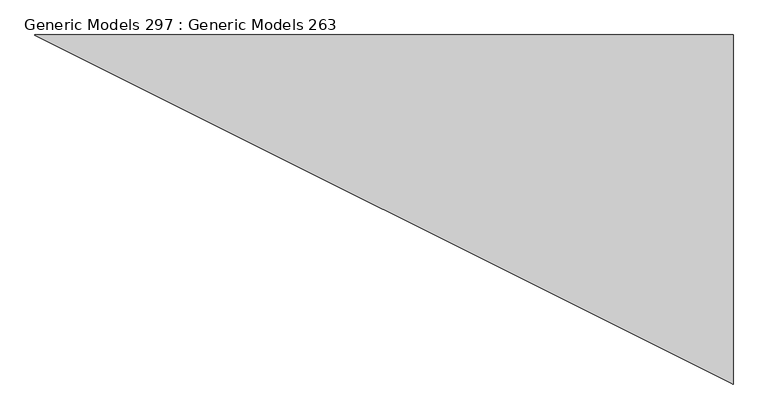
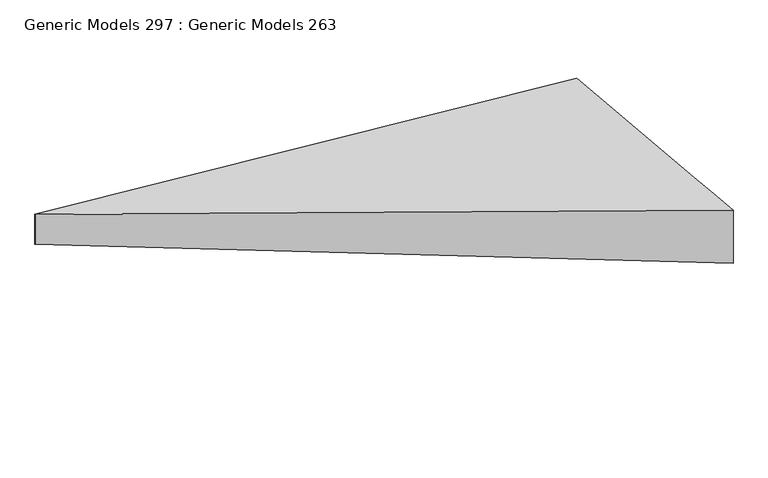
"""IFC4 building model written with IfcOpenShell, lengths in millimetres: proxy geometry, Generic Models 297 : Generic Models 263."""

import ifcopenshell
import ifcopenshell.guid

model = None  # the IFC model being written
_history = None  # IfcOwnerHistory: only IFC2X3 demands one
_inside = {}  # id of a spatial element -> (the spatial element, [elements in it])
_under = {}  # id of a project, library or spatial element -> (it, [spatial elements below it])
_declared = {}  # id of a project -> (the project, [libraries it declares])
_typed = {}  # id of a type object -> (the type object, [elements of that type])
_made_of = {}  # id of a material, layer set ... -> (it, [elements and type objects made of it])


def new_model(schema):
    """Start an empty IFC model of exactly this schema.

    Asked for "IFC4X3", IfcOpenShell would pick the latest addendum, in which some entities
    have other attributes; the version numbers below select the first issue.
    IFC2X3 requires an IfcOwnerHistory on every rooted entity: one is made here for all.
    """
    global model, _history
    if schema == "IFC4X3":
        model = ifcopenshell.file(schema_version=(4, 3, 0, 0))
    else:
        model = ifcopenshell.file(schema=schema)
    _inside.clear()
    _under.clear()
    _declared.clear()
    _typed.clear()
    _made_of.clear()
    _history = None
    if model.schema == "IFC2X3":
        org = make("IfcOrganization", Name="unknown")
        user = make(
            "IfcPersonAndOrganization",
            ThePerson=make("IfcPerson", FamilyName="unknown"),
            TheOrganization=org,
        )
        app = make(
            "IfcApplication",
            ApplicationDeveloper=org,
            Version="unknown",
            ApplicationFullName="unknown",
            ApplicationIdentifier="unknown",
        )
        _history = make(
            "IfcOwnerHistory",
            OwningUser=user,
            OwningApplication=app,
            ChangeAction="ADDED",
            CreationDate=0,
        )
    return model


def make(cls, **values):
    """One entity of the class cls with the attributes given. An attribute that is None is left unset."""
    return model.create_entity(
        cls, **{name: value for name, value in values.items() if value is not None}
    )


def rooted(cls, **values):
    """An entity with a GlobalId (a new one), such as an element, a storey or a relation."""
    return make(cls, GlobalId=ifcopenshell.guid.new(), OwnerHistory=_history, **values)


def si_unit(unit_type, name, prefix=None):
    """IfcSIUnit, for example si_unit("LENGTHUNIT", "METRE", prefix="MILLI")."""
    return make("IfcSIUnit", UnitType=unit_type, Prefix=prefix, Name=name)


def assignment(units):
    """IfcUnitAssignment: the units of a project."""
    return None if units is None else make("IfcUnitAssignment", Units=units)


def point(xyz):
    """IfcCartesianPoint."""
    return None if xyz is None else make("IfcCartesianPoint", Coordinates=xyz)


def direction(xyz):
    """IfcDirection."""
    return None if xyz is None else make("IfcDirection", DirectionRatios=xyz)


def frame(location, z_axis=None, x_axis=None):
    """IfcAxis2Placement3D, a coordinate frame: its origin and axes. An axis left out is left unset."""
    return make(
        "IfcAxis2Placement3D",
        Location=point(location),
        Axis=direction(z_axis),
        RefDirection=direction(x_axis),
    )


def origin():
    """The frame at (0, 0, 0) with its axes left unset."""
    return frame((0.0, 0.0, 0.0))


def place(relative_to, where):
    """IfcLocalPlacement: puts the frame where relative to a parent placement (None: the world)."""
    return make(
        "IfcLocalPlacement", PlacementRelTo=relative_to, RelativePlacement=where
    )


def context(
    kind, dimensions, precision=None, world=None, true_north=None, identifier=None
):
    """IfcGeometricRepresentationContext, for example the 3D "Model" context."""
    return make(
        "IfcGeometricRepresentationContext",
        ContextIdentifier=identifier,
        ContextType=kind,
        CoordinateSpaceDimension=dimensions,
        Precision=precision,
        WorldCoordinateSystem=world,
        TrueNorth=true_north,
    )


def project(units=None, contexts=None):
    """IfcProject with its units and contexts."""
    return rooted(
        "IfcProject",
        Name="project",
        RepresentationContexts=contexts,
        UnitsInContext=assignment(units),
    )


def spatial(cls, under=None, at=None, **own):
    """A site, building, storey or space (cls), placed at a placement, below another one or the project."""
    s = rooted(cls, ObjectPlacement=at, **own)
    if under is not None:
        _under.setdefault(under.id(), (under, []))[1].append(s)
    return s


def shape(context_of_items, identifier, shape_type, items):
    """IfcShapeRepresentation: the items that make up one representation, for example the "Body"."""
    return make(
        "IfcShapeRepresentation",
        ContextOfItems=context_of_items,
        RepresentationIdentifier=identifier,
        RepresentationType=shape_type,
        Items=items,
    )


def source(mapping_origin, context_of_items, identifier, shape_type, items):
    """IfcRepresentationMap: a shape defined once, which mapped items show again and again."""
    return make(
        "IfcRepresentationMap",
        MappingOrigin=mapping_origin,
        MappedRepresentation=shape(context_of_items, identifier, shape_type, items),
    )


def transform(
    local_origin,
    x_axis=None,
    y_axis=None,
    z_axis=None,
    scale=None,
    scale2=None,
    scale3=None,
    uniform=True,
):
    """IfcCartesianTransformationOperator3D, or its non-uniform kind. x_axis, y_axis, z_axis: its Axis1, 2, 3."""
    if uniform:
        return make(
            "IfcCartesianTransformationOperator3D",
            Axis1=direction(x_axis),
            Axis2=direction(y_axis),
            LocalOrigin=point(local_origin),
            Scale=scale,
            Axis3=direction(z_axis),
        )
    return make(
        "IfcCartesianTransformationOperator3DnonUniform",
        Axis1=direction(x_axis),
        Axis2=direction(y_axis),
        LocalOrigin=point(local_origin),
        Scale=scale,
        Axis3=direction(z_axis),
        Scale2=scale2,
        Scale3=scale3,
    )


def mapped(mapping_source, mapping_target):
    """IfcMappedItem: shows the shape of a source again, moved by a transform."""
    return make(
        "IfcMappedItem", MappingSource=mapping_source, MappingTarget=mapping_target
    )


def made_of(thing, what):
    """Note that an element or type object is made of a material, layer set ...; save() writes the relation."""
    if what is not None:
        _made_of.setdefault(what.id(), (what, []))[1].append(thing)
    return thing


def element(
    cls,
    number,
    at=None,
    inside=None,
    cuts=None,
    type_object=None,
    material=None,
    context=None,
    identifier="Body",
    shape_type=None,
    held_by="IfcProductDefinitionShape",
    body=None,
    shapes=None,
    **own,
):
    """One element of the class cls, such as IfcWall. Its Tag is "e" and its number.

    at: its placement. inside: the storey or other place that contains it. cuts: it is an
    opening in that element (IfcRelVoidsElement). A single representation is given by context,
    identifier, shape_type and body (its items); several are given by shapes. held_by: the class
    of the entity that holds the representations. save() writes the other relations.
    """
    e = rooted(cls, Tag="e%d" % number, ObjectPlacement=at, **own)
    if body is not None:
        shapes = [shape(context, identifier, shape_type, body)]
    if shapes is not None:
        e.Representation = make(held_by, Representations=shapes)
    if inside is not None:
        _inside.setdefault(inside.id(), (inside, []))[1].append(e)
    if cuts is not None:
        rooted(
            "IfcRelVoidsElement", RelatingBuildingElement=cuts, RelatedOpeningElement=e
        )
    if type_object is not None:
        _typed.setdefault(type_object.id(), (type_object, []))[1].append(e)
    return made_of(e, material)


def aggregate(whole, parts):
    """IfcRelAggregates: a whole, such as a stair, and the parts it consists of."""
    return rooted("IfcRelAggregates", RelatingObject=whole, RelatedObjects=parts)


def save(model, path):
    """Write the relations noted so far, then the file.

    IfcRelAggregates (storeys below a building ...), IfcRelContainedInSpatialStructure (elements
    in a storey), IfcRelDefinesByType, IfcRelAssociatesMaterial and IfcRelDeclares: one each for
    every whole, place, type object, material and project.
    """
    for whole, parts in _under.values():
        aggregate(whole, parts)
    for where, things in _inside.values():
        rooted(
            "IfcRelContainedInSpatialStructure",
            RelatedElements=things,
            RelatingStructure=where,
        )
    for kind, things in _typed.values():
        rooted("IfcRelDefinesByType", RelatedObjects=things, RelatingType=kind)
    for what, things in _made_of.values():
        rooted("IfcRelAssociatesMaterial", RelatedObjects=things, RelatingMaterial=what)
    for by, libraries in _declared.values():
        rooted("IfcRelDeclares", RelatingContext=by, RelatedDefinitions=libraries)
    model.write(path)


def plane_surface(at):
    """IfcPlane: the flat surface through the origin of the frame at, square to its z axis."""
    return make("IfcPlane", Position=at)


def spline_surface(u_degree, v_degree, points, u_multiplicities, v_multiplicities, u_knots, v_knots, weights=None):
    """IfcBSplineSurfaceWithKnots; with weights, IfcRationalBSplineSurfaceWithKnots. points: one row for each step in u."""
    own = dict(
        UDegree=u_degree,
        VDegree=v_degree,
        ControlPointsList=[[point(p) for p in row] for row in points],
        SurfaceForm="UNSPECIFIED",
        UClosed=False,
        VClosed=False,
        SelfIntersect=False,
        UMultiplicities=u_multiplicities,
        VMultiplicities=v_multiplicities,
        UKnots=u_knots,
        VKnots=v_knots,
        KnotSpec="UNSPECIFIED",
    )
    if weights is None:
        return make("IfcBSplineSurfaceWithKnots", **own)
    return make("IfcRationalBSplineSurfaceWithKnots", WeightsData=weights, **own)


def advanced_brep(points, edges, surfaces, faces):
    """IfcAdvancedBrep: a solid bounded by faces that lie on surfaces and meet in shared edges.

    An edge is (start, end): straight between two places in points (the first is 0);
    or (start, end, curve); or (start, end, curve, False) where it runs against its curve.
    A face is (place in surfaces, loops), or (place, loops, False) where it looks against
    its surface's normal. A loop lists edges by number (the first is 1), with a minus sign
    where the edge is run from its end to its start. The first loop is the outer one.
    """
    corners = [point(p) for p in points]
    vertices = [make("IfcVertexPoint", VertexGeometry=c) for c in corners]
    made = []
    for start, end, *more in edges:
        made.append(
            make(
                "IfcEdgeCurve",
                EdgeStart=vertices[start],
                EdgeEnd=vertices[end],
                EdgeGeometry=more[0] if more else make("IfcPolyline", Points=[corners[start], corners[end]]),
                SameSense=more[1] if len(more) > 1 else True,
            )
        )
    hull = []
    for where, loops, *sense in faces:
        bounds = []
        for j, loop in enumerate(loops):
            ring = [make("IfcOrientedEdge", EdgeElement=made[abs(k) - 1], Orientation=k > 0) for k in loop]
            bounds.append(
                make(
                    "IfcFaceOuterBound" if j == 0 else "IfcFaceBound",
                    Bound=make("IfcEdgeLoop", EdgeList=ring),
                    Orientation=True,
                )
            )
        hull.append(make("IfcAdvancedFace", Bounds=bounds, FaceSurface=surfaces[where], SameSense=sense[0] if sense else True))
    return make("IfcAdvancedBrep", Outer=make("IfcClosedShell", CfsFaces=hull))


def generic_models_297_generic_models_263_bc1a45ca(model_context):
    return source(origin(), model_context, "Body", "AdvancedBrep", [
        advanced_brep(
        [(91554.5797726, -8256.6272578, 2.0699085), (91554.5797726, -8256.6272578, -314.8198762), (91554.5797726, -6732.6272578, -314.8198762), (91554.5797726, -6732.6272578, -137.0198762), (88506.5797726, -6733.7737439, 120.3150753), (88506.5797726, -6732.6272578, 120.3150753), (88506.5797726, -6732.6272578, -58.1173502), (88506.5797726, -6733.7737439, -58.1173502)],
        [
            (0, 1),
            (1, 2),
            (2, 3),
            (3, 0),
            (4, 5),
            (5, 6),
            (6, 7),
            (7, 4),
            (7, 1),
            (0, 4),
            (6, 2),
            (5, 3),
        ],
        [
            plane_surface(frame((91554.5797726, -7494.6272578, -191.14743), z_axis=(1.0, 0.0, 0.0), x_axis=(0.0, 0.0, -1.0))),
            plane_surface(frame((88506.5797726, -6733.2005009, 31.0988625), z_axis=(-1.0, 0.0, 0.0), x_axis=(0.0, 0.0, -1.0))),
            plane_surface(frame((88506.5797726, -6733.7737439, 31.0988625), z_axis=(-0.4469443881993885, -0.894561744016071, 0.0), x_axis=(0.0, 0.0, -1.0))),
            plane_surface(frame((88506.5797726, -6733.2005009, -58.1173502), z_axis=(-0.08392288197547094, 0.0, -0.9964722524390387), x_axis=(0.0, 1.0, 0.0))),
            plane_surface(frame((88506.5797726, -6732.6272578, 31.0988625), z_axis=(0.0, 1.0, 0.0), x_axis=(0.0, 0.0, 1.0))),
            spline_surface(1, 1, [[(88506.5797726, -6732.6272578, 120.3150753), (91554.5797726, -6732.6272578, -137.0198762)], [(88506.5797726, -6733.7737439, 120.3150753), (91554.5797726, -8256.6272578, 2.0699085)]], [2, 2], [2, 2], [0.0, 1.0], [0.0, 1.0]),
        ],
        [
            (0, [[1, 2, 3, 4]]),
            (1, [[5, 6, 7, 8]]),
            (2, [[-8, 9, -1, 10]]),
            (3, [[-7, 11, -2, -9]]),
            (4, [[-6, 12, -3, -11]]),
            (5, [[-5, -10, -4, -12]]),
        ],
    ),
    ])


if __name__ == "__main__":
    model = new_model("IFC4")
    model_context = context("Model", 3, world=origin())
    ifc_project = project(units=[si_unit("LENGTHUNIT", "METRE", prefix="MILLI")], contexts=[model_context])
    site = spatial("IfcSite", under=ifc_project)
    building = spatial("IfcBuilding", under=site)
    placement = place(None, origin())
    generic_models_297_generic_models_263_shape = generic_models_297_generic_models_263_bc1a45ca(model_context)
    element("IfcBuildingElementProxy", 1, Name="Generic Models 297 : Generic Models 263", ObjectType="Generic Models 297 : Generic Models 263", at=placement, inside=building, context=model_context, shape_type="MappedRepresentation", body=[
        mapped(generic_models_297_generic_models_263_shape, transform((0.0, 0.0, 0.0), x_axis=(1.0, 0.0, 0.0), y_axis=(0.0, 1.0, 0.0), z_axis=(0.0, 0.0, 1.0))),
    ])
    save(model, "model.ifc")

# Revit data of these elements
# Element 1 (IfcBuildingElementProxy, "Generic Models 297 : Generic Models 263")
#   Materials on its faces: "SLOPED - 7\" CONC."
# Materials
#   "SLOPED - 7\" CONC.": class "Concrete", colour RGB 191 191 191, transparency 0, Description = "Cast-in-place concrete", Cost = 0
